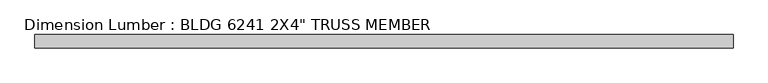
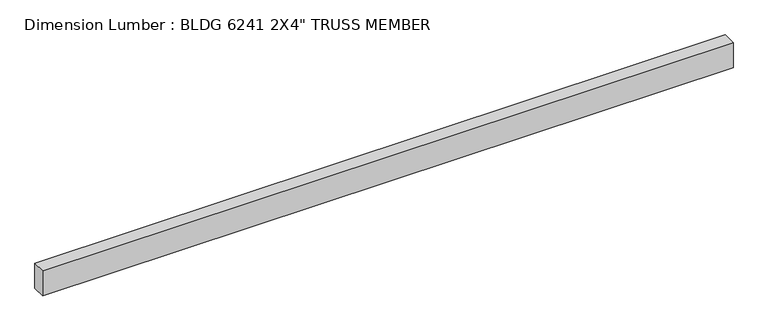
"""IFC4 building model written with IfcOpenShell, lengths in millimetres: beam geometry."""

from ifc_helpers import new_model, si_unit, frame, origin, place, context, project, spatial, polyline, outline, extrude, source, transform, mapped, element, save


def beam_35a73032(model_context):
    return source(origin(), model_context, "Body", "SweptSolid", [
        extrude(outline(polyline([(1320.8, 25.4), (1320.8, -25.4), (-1320.8, -25.4), (-1320.8, 25.4), (1320.8, 25.4)])), frame((0.0, 0.0, -50.8), z_axis=(0.0, 0.0, 1.0), x_axis=(1.0, 0.0, 0.0)), (0.0, 0.0, 1.0), 101.6),
    ])


if __name__ == "__main__":
    model = new_model("IFC4")
    model_context = context("Model", 3, world=origin())
    ifc_project = project(units=[si_unit("LENGTHUNIT", "METRE", prefix="MILLI")], contexts=[model_context])
    site = spatial("IfcSite", under=ifc_project)
    building = spatial("IfcBuilding", under=site)
    placement = place(None, origin())
    beam_shape = beam_35a73032(model_context)
    element("IfcBeam", 1, ObjectType="Dimension Lumber : BLDG 6241 2X4\" TRUSS MEMBER", at=placement, inside=building, context=model_context, shape_type="MappedRepresentation", body=[
        mapped(beam_shape, transform((0.0, 0.0, 0.0), x_axis=(1.0, 0.0, 0.0), y_axis=(0.0, 1.0, 0.0), z_axis=(0.0, 0.0, 1.0))),
    ])
    save(model, "model.ifc")

# Revit data of these elements
# Type "Dimension Lumber : BLDG 6241 2X4\" TRUSS MEMBER"
#   Assembly Code = "B10"
#   A = 0.273472 SF
#   Length [instance default] = 5' - 0"
#   b = 0' - 2"
#   d = 0' - 4"
#   Structural Material [instance default] = Softwood, Lumber
# Element 1 (IfcBeam, "Dimension Lumber : BLDG 6241 2X4\" TRUSS MEMBER")
#   Materials on its faces: "Softwood, Lumber"
# Materials
#   "Softwood, Lumber": class "Wood", colour RGB 223 192 134, transparency 0, Description = "Pinus Echinata", Cost = 0
